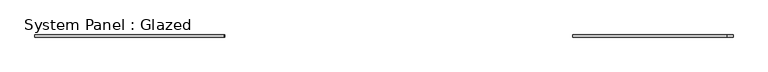
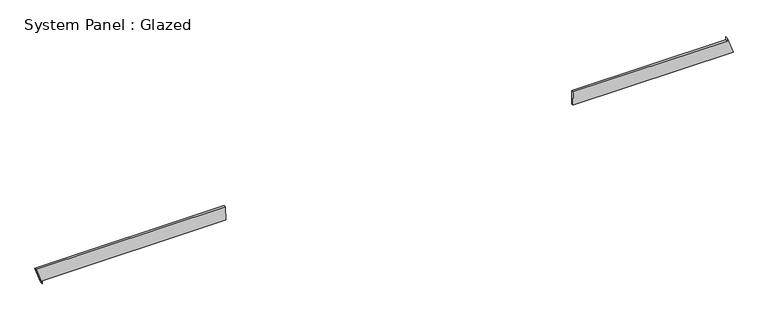
"""IFC4 building model written with IfcOpenShell, lengths in millimetres: plate geometry, System Panel : Glazed."""

from ifc_helpers import new_model, si_unit, frame, origin, place, context, project, spatial, polyline, outline, extrude, source, transform, mapped, element, save


def system_panel_glazed_7d35821c(model_context):
    return source(origin(), model_context, "Body", "SweptSolid", [
        extrude(outline(polyline([(0.0, -3956.9172633), (35.3553391, -3956.9172633), (35.3553391, -1838.1624938), (198.8114469, -1840.6577735), (198.8112207, -4026.9889068), (0.0, -3956.9172633)])), frame((0.0, -49.5, 0.0), z_axis=(0.0, 1.0, 0.0), x_axis=(0.0, 0.0, 1.0)), (0.0, 0.0, 1.0), 25.0),
        extrude(outline(polyline([(35.3553391, 2176.8405043), (35.3553391, 4026.9889068), (234.167386, 3956.9192133), (198.8120469, 3956.919217), (198.811863, 2179.8028801), (35.3553391, 2176.8405043)])), frame((0.0, -49.5, 0.0), z_axis=(0.0, 1.0, 0.0), x_axis=(0.0, 0.0, 1.0)), (0.0, 0.0, 1.0), 25.0),
    ])


if __name__ == "__main__":
    model = new_model("IFC4")
    model_context = context("Model", 3, world=origin())
    ifc_project = project(units=[si_unit("LENGTHUNIT", "METRE", prefix="MILLI")], contexts=[model_context])
    site = spatial("IfcSite", under=ifc_project)
    building = spatial("IfcBuilding", under=site)
    placement = place(None, origin())
    system_panel_glazed_shape = system_panel_glazed_7d35821c(model_context)
    element("IfcPlate", 1, ObjectType="System Panel : Glazed", at=placement, inside=building, context=model_context, shape_type="MappedRepresentation", body=[
        mapped(system_panel_glazed_shape, transform((0.0, 0.0, 0.0), x_axis=(1.0, 0.0, 0.0), y_axis=(0.0, 1.0, 0.0), z_axis=(0.0, 0.0, 1.0))),
    ])
    save(model, "model.ifc")

# Revit data of these elements
# Element 1 (IfcPlate, "System Panel : Glazed")
#   Materials on its faces: "Glass"
# Materials
#   "Glass": class "Glass", colour RGB 218 227 224, transparency 0.85, Description = "Soda Lime Glass", Cost = 0
